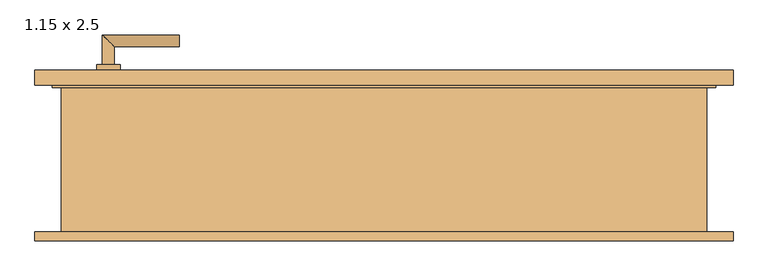
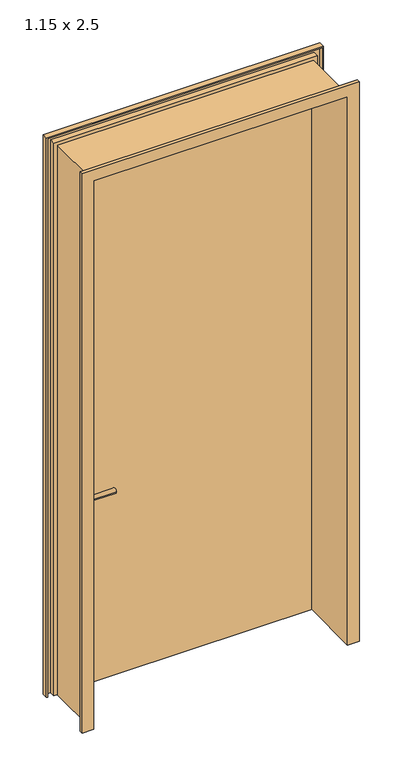
"""IFC4 building model written with IfcOpenShell, lengths in millimetres: door geometry, Drehflügel 1-flg - Stahlzarge : 1.15 x 2.5."""

from ifc_helpers import new_model, si_unit, point, frame, frame_2d, origin, place, context, project, spatial, polyline, circle_curve, ellipse_curve, trimmed, segment, composite_curve, outline, extrude, faceted_brep, source, transform, mapped, element, save
from ifc_brep_helpers import plane_surface, cylinder_surface, advanced_brep


def door_1_15_x_2_5_5b8efd12(model_context):
    return source(origin(), model_context, "Body", "SolidModel", [
        advanced_brep(
        [(-477.5, 114.4346141, 901.0), (-457.5, 114.4346141, 901.0), (-477.5, 44.4346141, 901.0), (-457.5, 64.4346141, 901.0), (-347.5, 44.4346141, 901.0), (-347.5, 64.4346141, 901.0)],
        [
            (0, 1, circle_curve(frame((-467.5, 114.4346141, 901.0), z_axis=(0.0, 1.0, 0.0), x_axis=(1.0, 0.0, 0.0)), 10.0)),
            (1, 0, circle_curve(frame((-467.5, 114.4346141, 901.0), z_axis=(0.0, 1.0, 0.0), x_axis=(1.0, 0.0, 0.0)), 10.0)),
            (0, 2),
            (2, 3, ellipse_curve(frame((-467.5, 54.4346141, 901.0), z_axis=(-0.7071067811865385, 0.7071067811865565, 0.0), x_axis=(0.7071067811865563, 0.7071067811865386, 0.0)), 14.1421356, 10.0)),
            (3, 1),
            (3, 2, ellipse_curve(frame((-467.5, 54.4346141, 901.0), z_axis=(-0.7071067811865385, 0.7071067811865565, 0.0), x_axis=(0.7071067811865563, 0.7071067811865386, 0.0)), 14.1421356, 10.0)),
            (4, 5, circle_curve(frame((-347.5, 54.4346141, 901.0), z_axis=(1.0, 0.0, 0.0), x_axis=(0.0, 1.0, 0.0)), 10.0)),
            (5, 4, circle_curve(frame((-347.5, 54.4346141, 901.0), z_axis=(1.0, 0.0, 0.0), x_axis=(0.0, 1.0, 0.0)), 10.0)),
            (2, 4),
            (5, 3),
        ],
        [
            plane_surface(frame((-467.5, 114.4346141, -386.7526403), z_axis=(0.0, 1.0, 0.0), x_axis=(0.0, 0.0, 1.0))),
            cylinder_surface(frame((-467.5, 114.4346141, 901.0), z_axis=(0.0, 1.0, 0.0), x_axis=(1.0, 0.0, 0.0)), 10.0),
            plane_surface(frame((-347.5, 54.4346141, -386.7526403), z_axis=(1.0, 0.0, 0.0), x_axis=(0.0, 0.0, 1.0))),
            cylinder_surface(frame((-467.5, 54.4346141, 901.0), z_axis=(-1.0, 0.0, 0.0), x_axis=(0.0, 1.0, 0.0)), 10.0),
        ],
        [
            (0, [[1, 2]]),
            (1, [[-1, 3, 4, 5]]),
            (1, [[-2, -5, 6, -3]]),
            (2, [[7, 8]]),
            (3, [[-4, 9, -8, 10]]),
            (3, [[-6, -10, -7, -9]]),
        ],
    ),
        advanced_brep(
        [(-457.5, 174.4346141, 901.0), (-477.5, 174.4346141, 901.0), (-457.5, 204.4346141, 901.0), (-477.5, 224.4346141, 901.0), (-347.5, 204.4346141, 901.0), (-347.5, 224.4346141, 901.0)],
        [
            (0, 1, circle_curve(frame((-467.5, 174.4346141, 901.0), z_axis=(0.0, -1.0, 0.0), x_axis=(-1.0, 0.0, 0.0)), 10.0)),
            (1, 0, circle_curve(frame((-467.5, 174.4346141, 901.0), z_axis=(0.0, -1.0, 0.0), x_axis=(-1.0, 0.0, 0.0)), 10.0)),
            (0, 2),
            (2, 3, ellipse_curve(frame((-467.5, 214.4346141, 901.0), z_axis=(-0.7071067811865475, -0.7071067811865475, 0.0), x_axis=(0.7071067811865474, -0.7071067811865476, 0.0)), 14.1421356, 10.0)),
            (3, 1),
            (3, 2, ellipse_curve(frame((-467.5, 214.4346141, 901.0), z_axis=(-0.7071067811865475, -0.7071067811865475, 0.0), x_axis=(0.7071067811865474, -0.7071067811865476, 0.0)), 14.1421356, 10.0)),
            (4, 5, circle_curve(frame((-347.5, 214.4346141, 901.0), z_axis=(1.0, 0.0, 0.0), x_axis=(0.0, 1.0, 0.0)), 10.0)),
            (5, 4, circle_curve(frame((-347.5, 214.4346141, 901.0), z_axis=(1.0, 0.0, 0.0), x_axis=(0.0, 1.0, 0.0)), 10.0)),
            (2, 4),
            (5, 3),
        ],
        [
            plane_surface(frame((-467.5, 174.4346141, -386.7526403), z_axis=(0.0, -1.0, 0.0), x_axis=(0.0, 0.0, 1.0))),
            cylinder_surface(frame((-467.5, 174.4346141, 901.0), z_axis=(0.0, -1.0, 0.0), x_axis=(-1.0, 0.0, 0.0)), 10.0),
            plane_surface(frame((-347.5, 214.4346141, -386.7526403), z_axis=(1.0, 0.0, 0.0), x_axis=(0.0, 0.0, 1.0))),
            cylinder_surface(frame((-467.5, 214.4346141, 901.0), z_axis=(-1.0, 0.0, 0.0), x_axis=(0.0, 1.0, 0.0)), 10.0),
        ],
        [
            (0, [[1, 2]]),
            (1, [[-1, 3, 4, 5]]),
            (1, [[-2, -5, 6, -3]]),
            (2, [[7, 8]]),
            (3, [[-4, 9, -8, 10]]),
            (3, [[-6, -10, -7, -9]]),
        ],
    ),
        extrude(outline(composite_curve([segment(trimmed(circle_curve(frame_2d((901.0, -467.5)), 20.0), [point((901.0, -487.5))], [point((901.0, -447.5))], False, "CARTESIAN"), True, "CONTINUOUS"), segment(trimmed(circle_curve(frame_2d((901.0, -467.5)), 20.0), [point((901.0, -447.5))], [point((901.0, -487.5))], False, "CARTESIAN"), True, "CONTINUOUS")], self_intersect=False)), frame((0.0, 104.4346141, 0.0), z_axis=(0.0, 1.0, 0.0), x_axis=(0.0, 0.0, 1.0)), (0.0, 0.0, 1.0), 10.0),
        extrude(outline(composite_curve([segment(trimmed(circle_curve(frame_2d((901.0, -467.5)), 20.0), [point((901.0, -487.5))], [point((901.0, -447.5))], False, "CARTESIAN"), True, "CONTINUOUS"), segment(trimmed(circle_curve(frame_2d((901.0, -467.5)), 20.0), [point((901.0, -447.5))], [point((901.0, -487.5))], False, "CARTESIAN"), True, "CONTINUOUS")], self_intersect=False)), frame((0.0, 164.4346141, 0.0), z_axis=(0.0, 1.0, 0.0), x_axis=(0.0, 0.0, 1.0)), (0.0, 0.0, 1.0), 10.0),
        extrude(outline(polyline([(557.5, 139.4346141), (-557.5, 139.4346141), (-557.5, 164.4346141), (557.5, 164.4346141), (557.5, 139.4346141)])), frame((0.0, 0.0, 1.0), z_axis=(0.0, 0.0, 1.0), x_axis=(1.0, 0.0, 0.0)), (0.0, 0.0, 1.0), 2490.0),
        faceted_brep([(591.9603207, -125.5653859, 1.0), (542.5, -125.5653859, 1.0), (542.5, 139.4346141, 1.0), (557.5, 139.4346141, 1.0), (557.5, 164.4346141, 1.0), (591.9603207, 164.4346141, 1.0), (591.9603207, 139.4346141, 1.0), (586.9603207, 139.4346141, 1.0), (586.9603207, 159.4346141, 1.0), (562.5, 159.4346141, 1.0), (562.5, 134.4346141, 1.0), (547.5, 134.4346141, 1.0), (547.5, -120.5653859, 1.0), (586.9603207, -120.5653859, 1.0), (586.9603207, -110.5653859, 1.0), (591.9603207, -110.5653859, 1.0), (591.9603207, -125.5653859, 2525.4603207), (-591.9603207, -125.5653859, 2525.4603207), (-591.9603207, -125.5653859, 1.0), (-542.5, -125.5653859, 1.0), (-542.5, -125.5653859, 2476.0), (542.5, -125.5653859, 2476.0), (542.5, 139.4346141, 2476.0), (-542.5, 139.4346141, 2476.0), (-542.5, 139.4346141, 1.0), (-557.5, 139.4346141, 1.0), (-557.5, 139.4346141, 2491.0), (557.5, 139.4346141, 2491.0), (557.5, 164.4346141, 2491.0), (-557.5, 164.4346141, 2491.0), (-557.5, 164.4346141, 1.0), (-591.9603207, 164.4346141, 1.0), (-591.9603207, 164.4346141, 2525.4603207), (591.9603207, 164.4346141, 2525.4603207), (591.9603207, 139.4346141, 2525.4603207), (-591.9603207, 139.4346141, 2525.4603207), (-591.9603207, 139.4346141, 1.0), (-586.9603207, 139.4346141, 1.0), (-586.9603207, 139.4346141, 2520.4603207), (586.9603207, 139.4346141, 2520.4603207), (586.9603207, 159.4346141, 2520.4603207), (-586.9603207, 159.4346141, 2520.4603207), (-586.9603207, 159.4346141, 1.0), (-562.5, 159.4346141, 1.0), (-562.5, 159.4346141, 2496.0), (562.5, 159.4346141, 2496.0), (562.5, 134.4346141, 2496.0), (-562.5, 134.4346141, 2496.0), (-562.5, 134.4346141, 1.0), (-547.5, 134.4346141, 1.0), (-547.5, 134.4346141, 2481.0), (547.5, 134.4346141, 2481.0), (547.5, -120.5653859, 2481.0), (-547.5, -120.5653859, 2481.0), (-547.5, -120.5653859, 1.0), (-586.9603207, -120.5653859, 1.0), (-586.9603207, -120.5653859, 2520.4603207), (586.9603207, -120.5653859, 2520.4603207), (586.9603207, -110.5653859, 2520.4603207), (-586.9603207, -110.5653859, 2520.4603207), (-586.9603207, -110.5653859, 1.0), (-591.9603207, -110.5653859, 1.0), (-591.9603207, -110.5653859, 2525.4603207), (591.9603207, -110.5653859, 2525.4603207)], [[[0, 1, 2, 3, 4, 5, 6, 7, 8, 9, 10, 11, 12, 13, 14, 15]], [[1, 0, 16, 17, 18, 19, 20, 21]], [[2, 1, 21, 22]], [[3, 2, 22, 23, 24, 25, 26, 27]], [[4, 3, 27, 28]], [[5, 4, 28, 29, 30, 31, 32, 33]], [[6, 5, 33, 34]], [[7, 6, 34, 35, 36, 37, 38, 39]], [[8, 7, 39, 40]], [[9, 8, 40, 41, 42, 43, 44, 45]], [[10, 9, 45, 46]], [[11, 10, 46, 47, 48, 49, 50, 51]], [[12, 11, 51, 52]], [[13, 12, 52, 53, 54, 55, 56, 57]], [[14, 13, 57, 58]], [[15, 14, 58, 59, 60, 61, 62, 63]], [[0, 15, 63, 16]], [[17, 62, 61, 18]], [[18, 61, 60, 55, 54, 49, 48, 43, 42, 37, 36, 31, 30, 25, 24, 19]], [[23, 20, 19, 24]], [[29, 26, 25, 30]], [[35, 32, 31, 36]], [[41, 38, 37, 42]], [[47, 44, 43, 48]], [[53, 50, 49, 54]], [[59, 56, 55, 60]], [[22, 21, 20, 23]], [[28, 27, 26, 29]], [[34, 33, 32, 35]], [[40, 39, 38, 41]], [[46, 45, 44, 47]], [[52, 51, 50, 53]], [[58, 57, 56, 59]], [[16, 63, 62, 17]]]),
    ])


if __name__ == "__main__":
    model = new_model("IFC4")
    model_context = context("Model", 3, world=origin())
    ifc_project = project(units=[si_unit("LENGTHUNIT", "METRE", prefix="MILLI")], contexts=[model_context])
    site = spatial("IfcSite", under=ifc_project)
    building = spatial("IfcBuilding", under=site)
    placement = place(None, origin())
    door_1_15_x_2_5_shape = door_1_15_x_2_5_5b8efd12(model_context)
    element("IfcDoor", 1, ObjectType="Drehflügel 1-flg - Stahlzarge : 1.15 x 2.5", at=placement, inside=building, context=model_context, shape_type="MappedRepresentation", body=[
        mapped(door_1_15_x_2_5_shape, transform((0.0, 0.0, 0.0), x_axis=(1.0, 0.0, 0.0), y_axis=(0.0, 1.0, 0.0), z_axis=(0.0, 0.0, 1.0))),
    ])
    save(model, "model.ifc")

# Revit data of these elements
# Type "Drehflügel 1-flg - Stahlzarge : 1.15 x 2.5"
#   Type Mark = "21"
#   Operation = "SingleSwingRight"
#   Keynote = "16.03"
#   Analytic Construction = "Metall"
#   Thermal Resistance (R) = 0.270117 (m²·K)/W
#   Heat Transfer Coefficient (U) = 3.7021 W/(m²·K)
#   Rough Width = 1.135 m
#   Rough Height [instance default] = 2.600 m
#   Höhe Türgriff [instance default] = 0.900 m
#   Height = 2.500 m
#   Fußbodenaufbau [instance default] = 0.100 m
#   Width = 1.135 m
#   Sichtbarkeit Sturzlinien [instance default] = yes
#   Türgriff auswählen [instance default] = element 221079
#   Türgriff [instance default] = none
#   Türflügel [instance default] = none
#   Rahmen/Pfosten [instance default] = Metall - Lackiert - Grau
#   Visual Light Transmittance = 0
#   Solar Heat Gain Coefficient = 0
#   Function = (empty or 0)
#   Wall Closure = (empty or 0)
# Element 1 (IfcDoor, "Drehflügel 1-flg - Stahlzarge : 1.15 x 2.5")
#   Rough Height = 2.501 m
#   Fußbodenaufbau = 0.001 m
#   Materials on its faces: "Metall - Lackiert - Grau", "Metall - Chrom", "Holz - Birke"
# Materials
#   "Metall - Lackiert - Grau": class "Farbe 1", colour RGB 98 98 98, transparency 0, Cost = 0
#   "Metall - Chrom": class "Metall", colour RGB 247 247 247, transparency 0, Cost = 0
#   "Holz - Birke": class "Holz", colour RGB 213 164 103, transparency 0, Cost = 0
